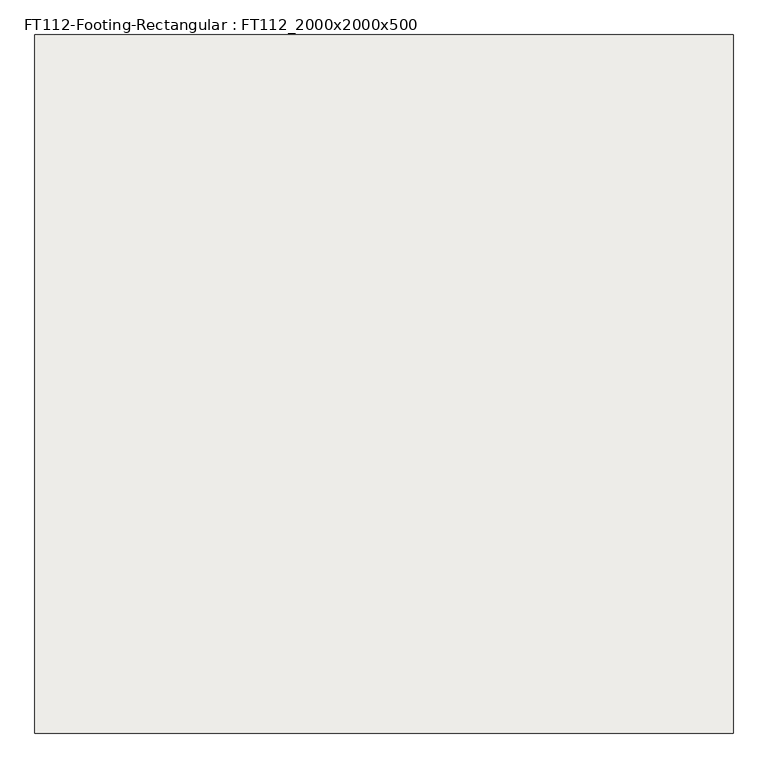
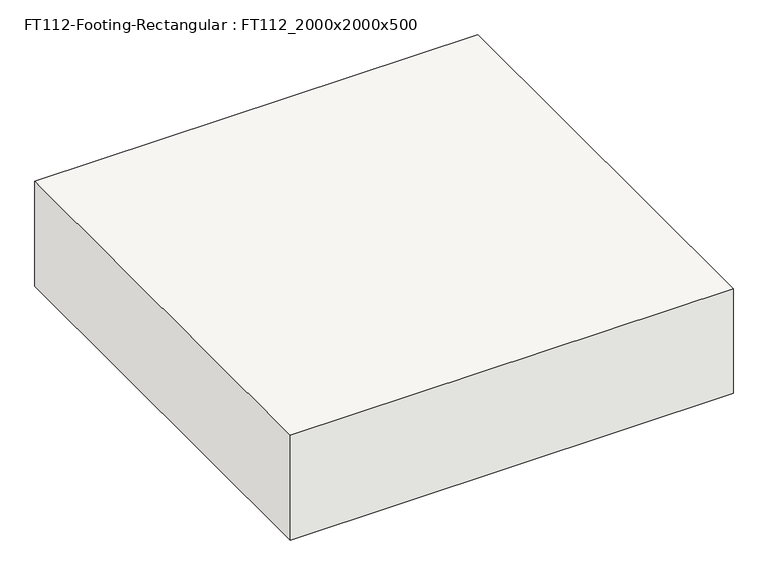
"""IFC4 building model written with IfcOpenShell, lengths in millimetres: slab geometry, FT112-Footing-Rectangular : FT112_2000x2000x500."""

from ifc_helpers import new_model, si_unit, frame, origin, place, context, project, spatial, polyline, outline, extrude, source, transform, mapped, element, save


def ft112_footing_rectangular_ft112_2000x2000x500_8ee35437(model_context):
    return source(origin(), model_context, "Body", "SweptSolid", [
        extrude(outline(polyline([(1000.0, 1000.0), (1000.0, -1000.0), (-1000.0, -1000.0), (-1000.0, 1000.0), (1000.0, 1000.0)])), frame((0.0, 0.0, -500.0), z_axis=(0.0, 0.0, 1.0), x_axis=(1.0, 0.0, 0.0)), (0.0, 0.0, 1.0), 500.0),
    ])


if __name__ == "__main__":
    model = new_model("IFC4")
    model_context = context("Model", 3, world=origin())
    ifc_project = project(units=[si_unit("LENGTHUNIT", "METRE", prefix="MILLI")], contexts=[model_context])
    site = spatial("IfcSite", under=ifc_project)
    building = spatial("IfcBuilding", under=site)
    placement = place(None, origin())
    ft112_footing_rectangular_ft112_2000x2000x500_shape = ft112_footing_rectangular_ft112_2000x2000x500_8ee35437(model_context)
    element("IfcSlab", 1, ObjectType="FT112-Footing-Rectangular : FT112_2000x2000x500", at=placement, inside=building, context=model_context, shape_type="MappedRepresentation", body=[
        mapped(ft112_footing_rectangular_ft112_2000x2000x500_shape, transform((0.0, 0.0, 0.0), x_axis=(1.0, 0.0, 0.0), y_axis=(0.0, 1.0, 0.0), z_axis=(0.0, 0.0, 1.0))),
    ])
    save(model, "model.ifc")

# Revit data of these elements
# Type "FT112-Footing-Rectangular : FT112_2000x2000x500"
#   Description = "UG Shallow Foundation"
#   Description = "UG Shallow Foundation"
#   Width = 2000 mm
#   Length = 2000 mm
#   Foundation Thickness = 500 mm
#   hec_material3 [instance default] = none
#   hec_material2 [instance default] = A03AE056-00001_Bitumen/Bituminous/Asphalt Coating
#   hec_material1 [instance default] = A03AC035-00001_Form Work (3 times in use)_Flat
#   Structural Material [instance default] = A03AC032-00007_Structural Concrete_Type1_25MPa-30Mpa
#   Assembly Code = ""
# Element 1 (IfcSlab, "FT112-Footing-Rectangular : FT112_2000x2000x500")
#   Structural Material = 콘크리트 - 현장타설 콘크리트
#   Materials on its faces: "콘크리트 - 현장타설 콘크리트"
# Materials
#   "A03AE056-00001_Bitumen/Bituminous/Asphalt Coating": class "Generic", colour RGB 17 17 17, transparency 0, Description = "Damp-proofing", W00) Work Master Code = "A03AE056-00001", W01) Work Master_Lv1 = "Concrete Work", W02) Work Master_Lv2 = "Concrete Protective Coating (U/G)", W03) Work Master_Spec.1 = "Bitumen/Bituminous/Asphalt Coating", Cost = 0
#   "A03AC035-00001_Form Work (3 times in use)_Flat": class "Wood", colour RGB 149 120 74, transparency 0, Description = "Plywood", W00) Work Master Code = "A03AC035-00001", W01) Work Master_Lv1 = "Concrete Work", W02) Work Master_Lv2 = "Substructure Work", W03) Work Master_Spec.1 = "Form Work (3 times in use)", W04) Work Master_Spec.2 = "Flat Form", W05) Work Master_Spec.3 = "Dressed Lumber, Plywood or Steel Form(Wood Planks are not Allowed) incl. Chamfer", Cost = 0
#   "A03AC032-00007_Structural Concrete_Type1_25MPa-30Mpa": class "Concrete", colour RGB 176 176 176, transparency 0, Keynote = "09910.A1", Description = "Reinf. Conc.", W00) Work Master Code = "A03AC032-00007", W01) Work Master_Lv1 = "Concrete Work", W02) Work Master_Lv2 = "Substructure Work", W03) Work Master_Spec.1 = "Structural Concrete", W04) Work Master_Spec.2 = "Cement Type-1", W05) Work Master_Spec.3 = "25MPa < F'c (Cylinder Strength) ≤ 30MPa", Cost = 0
#   "콘크리트 - 현장타설 콘크리트": class "콘크리트", colour RGB 192 192 192, transparency 0, Cost = 0
